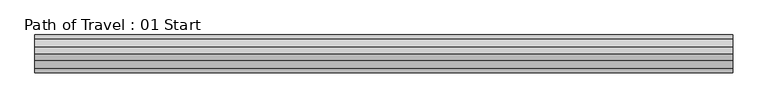
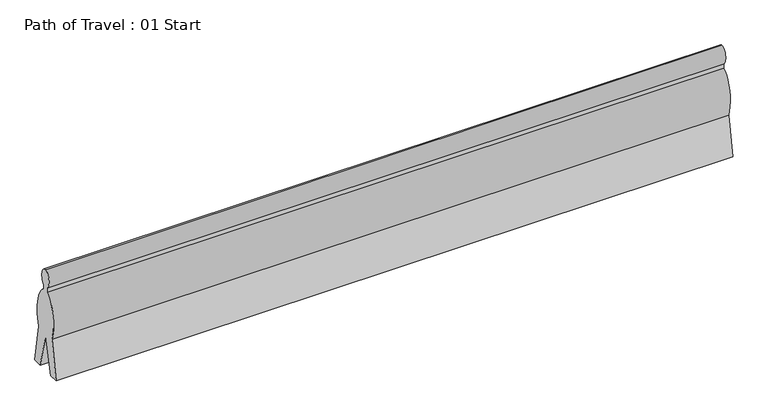
"""IFC4 building model written with IfcOpenShell, lengths in millimetres: proxy geometry, Path of Travel : 01 Start."""

from ifc_helpers import new_model, si_unit, point, frame, origin, place, context, project, spatial, ellipse_curve, trimmed, source, transform, mapped, element, save
from ifc_brep_helpers import plane_surface, extruded_surface, advanced_brep


def path_of_travel_01_start_212660b2(model_context):
    return source(origin(), model_context, "Body", "AdvancedBrep", [
        advanced_brep(
        [(227.5554837, 0.0, 1727.2), (227.5554837, 42.9018657, 1436.6534209), (227.5554837, 42.9018657, 1363.4763406), (227.5554837, 184.1186263, 643.4144547), (227.5554837, 297.5699544, 0.0), (227.5554837, 145.6574193, 0.0), (227.5554837, 0.0, 584.2), (227.5554837, -145.6574193, 0.0), (227.5554837, -297.5699544, 0.0), (227.5554837, -184.1186263, 643.4144547), (227.5554837, -42.9018657, 1363.4763406), (227.5554837, -42.9018657, 1436.6534209), (11200.3554837, 0.0, 1727.2), (11200.3554837, -42.9018657, 1436.6534209), (11200.3554837, -42.9018657, 1363.4763406), (11200.3554837, -184.1186263, 643.4144547), (11200.3554837, -297.5699544, 0.0), (11200.3554837, -145.6574193, 0.0), (11200.3554837, 0.0, 584.2), (11200.3554837, 145.6574193, 0.0), (11200.3554837, 297.5699544, 0.0), (11200.3554837, 184.1186263, 643.4144547), (11200.3554837, 42.9018657, 1363.4763406), (11200.3554837, 42.9018657, 1436.6534209)],
        [
            (0, 1, ellipse_curve(frame((227.5554837, 0.0, 1574.8), z_axis=(-1.0, 0.0, 0.0), x_axis=(0.0, 0.0, 1.0)), 152.4, 101.6)),
            (1, 2),
            (2, 3, ellipse_curve(frame((227.5554837, 0.0, 914.4), z_axis=(-1.0, 0.0, 0.0), x_axis=(0.0, 0.0, -1.0)), 457.2, 228.6)),
            (3, 4),
            (4, 5),
            (5, 6),
            (6, 7),
            (7, 8),
            (8, 9),
            (9, 10, ellipse_curve(frame((227.5554837, 0.0, 914.4), z_axis=(-1.0, 0.0, 0.0), x_axis=(0.0, 0.0, -1.0)), 457.2, 228.6)),
            (10, 11),
            (11, 0, ellipse_curve(frame((227.5554837, 0.0, 1574.8), z_axis=(-1.0, 0.0, 0.0), x_axis=(0.0, 0.0, 1.0)), 152.4, 101.6)),
            (12, 13, ellipse_curve(frame((11200.3554837, 0.0, 1574.8), z_axis=(1.0, 0.0, 0.0), x_axis=(0.0, 0.0, 1.0)), 152.4, 101.6)),
            (13, 14),
            (14, 15, ellipse_curve(frame((11200.3554837, 0.0, 914.4), z_axis=(1.0, 0.0, 0.0), x_axis=(0.0, 0.0, -1.0)), 457.2, 228.6)),
            (15, 16),
            (16, 17),
            (17, 18),
            (18, 19),
            (19, 20),
            (20, 21),
            (21, 22, ellipse_curve(frame((11200.3554837, 0.0, 914.4), z_axis=(1.0, 0.0, 0.0), x_axis=(0.0, 0.0, -1.0)), 457.2, 228.6)),
            (22, 23),
            (23, 12, ellipse_curve(frame((11200.3554837, 0.0, 1574.8), z_axis=(1.0, 0.0, 0.0), x_axis=(0.0, 0.0, 1.0)), 152.4, 101.6)),
            (0, 12),
            (23, 1),
            (22, 2),
            (21, 3),
            (20, 4),
            (19, 5),
            (18, 6),
            (17, 7),
            (16, 8),
            (15, 9),
            (14, 10),
            (13, 11),
        ],
        [
            plane_surface(frame((227.5554837, 0.0, 0.0), z_axis=(-1.0, 0.0, 0.0), x_axis=(0.0, 0.0, 1.0))),
            plane_surface(frame((11200.3554837, 0.0, 0.0), z_axis=(1.0, 0.0, 0.0), x_axis=(0.0, 0.0, 1.0))),
            extruded_surface(trimmed(ellipse_curve(frame((11200.3554837, 0.0, 1574.8), z_axis=(-1.0, 0.0, 0.0), x_axis=(0.0, 0.0, 1.0)), 152.4, 101.6), [point((11200.3554837, 0.0, 1727.2))], [point((11200.3554837, 42.9018657, 1436.6534209))], True, "CARTESIAN"), (-10972.8, 0.0, 0.0), 10972.8),
            plane_surface(frame((227.5554837, 42.9018657, 1436.6534209), z_axis=(0.0, 1.0, 0.0), x_axis=(1.0, 0.0, 0.0))),
            extruded_surface(trimmed(ellipse_curve(frame((11200.3554837, 0.0, 914.4), z_axis=(-1.0, 0.0, 0.0), x_axis=(0.0, 0.0, -1.0)), 457.2, 228.6), [point((11200.3554837, 42.9018657, 1363.4763406))], [point((11200.3554837, 184.1186263, 643.4144547))], True, "CARTESIAN"), (-10972.8, 0.0, 0.0), 10972.8),
            plane_surface(frame((227.5554837, 184.1186263, 643.4144547), z_axis=(0.0, 0.9848077530122078, 0.17364817766693205), x_axis=(1.0, 0.0, 0.0))),
            plane_surface(frame((227.5554837, 297.5699544, 0.0), z_axis=(0.0, 0.0, -1.0), x_axis=(1.0, 0.0, 0.0))),
            plane_surface(frame((227.5554837, 145.6574193, 0.0), z_axis=(0.0, -0.9702957262760199, -0.2419218955995739), x_axis=(1.0, 0.0, 0.0))),
            plane_surface(frame((227.5554837, 0.0, 584.2), z_axis=(0.0, 0.9702957262759961, -0.24192189559966923), x_axis=(1.0, 0.0, 0.0))),
            plane_surface(frame((227.5554837, -145.6574193, 0.0), z_axis=(0.0, 0.0, -1.0), x_axis=(1.0, 0.0, 0.0))),
            plane_surface(frame((227.5554837, -297.5699544, 0.0), z_axis=(0.0, -0.984807753012208, 0.17364817766693066), x_axis=(1.0, 0.0, 0.0))),
            extruded_surface(trimmed(ellipse_curve(frame((11200.3554837, 0.0, 914.4), z_axis=(-1.0, 0.0, 0.0), x_axis=(0.0, 0.0, -1.0)), 457.2, 228.6), [point((11200.3554837, -184.1186263, 643.4144547))], [point((11200.3554837, -42.9018657, 1363.4763406))], True, "CARTESIAN"), (-10972.8, 0.0, 0.0), 10972.8),
            plane_surface(frame((227.5554837, -42.9018657, 1363.4763406), z_axis=(0.0, -1.0, 0.0), x_axis=(1.0, 0.0, 0.0))),
            extruded_surface(trimmed(ellipse_curve(frame((11200.3554837, 0.0, 1574.8), z_axis=(-1.0, 0.0, 0.0), x_axis=(0.0, 0.0, 1.0)), 152.4, 101.6), [point((11200.3554837, -42.9018657, 1436.6534209))], [point((11200.3554837, 0.0, 1727.2))], True, "CARTESIAN"), (-10972.8, 0.0, 0.0), 10972.8),
        ],
        [
            (0, [[1, 2, 3, 4, 5, 6, 7, 8, 9, 10, 11, 12]]),
            (1, [[13, 14, 15, 16, 17, 18, 19, 20, 21, 22, 23, 24]]),
            (2, [[-1, 25, -24, 26]]),
            (3, [[-2, -26, -23, 27]]),
            (4, [[-3, -27, -22, 28]]),
            (5, [[-4, -28, -21, 29]]),
            (6, [[-5, -29, -20, 30]]),
            (7, [[-6, -30, -19, 31]]),
            (8, [[-7, -31, -18, 32]]),
            (9, [[-8, -32, -17, 33]]),
            (10, [[-9, -33, -16, 34]]),
            (11, [[-10, -34, -15, 35]]),
            (12, [[-11, -35, -14, 36]]),
            (13, [[-12, -36, -13, -25]]),
        ],
    ),
    ])


if __name__ == "__main__":
    model = new_model("IFC4")
    model_context = context("Model", 3, world=origin())
    ifc_project = project(units=[si_unit("LENGTHUNIT", "METRE", prefix="MILLI")], contexts=[model_context])
    site = spatial("IfcSite", under=ifc_project)
    building = spatial("IfcBuilding", under=site)
    placement = place(None, origin())
    path_of_travel_01_start_shape = path_of_travel_01_start_212660b2(model_context)
    element("IfcBuildingElementProxy", 1, Name="Path of Travel : 01 Start", ObjectType="Path of Travel : 01 Start", at=placement, inside=building, context=model_context, shape_type="MappedRepresentation", body=[
        mapped(path_of_travel_01_start_shape, transform((0.0, 0.0, 0.0), x_axis=(1.0, 0.0, 0.0), y_axis=(0.0, 1.0, 0.0), z_axis=(0.0, 0.0, 1.0))),
    ])
    save(model, "model.ifc")

# Revit data of these elements
# Type "Path of Travel : 01 Start"
#   Path of Egress [instance default] = 4' - 0"
#   built-in parameter 1001306 [instance default] = 4 (stored number, unit not read)
#   Dot at Start = yes
#   Arrow in Middle = yes
#   Arrow at End = no
#   Egress Path = none
# Element 1 (IfcBuildingElementProxy, "Path of Travel : 01 Start")
#   Path of Egress = 36' - 0"
#   built-in parameter 1001306 = 36 (stored number, unit not read)
#   Materials on its faces: "Egress Path Solid"
# Materials
#   "Egress Path Solid": class "Unassigned", colour RGB 255 128 64, transparency 0.75, Comments = "Rendering appearance not upgraded "
